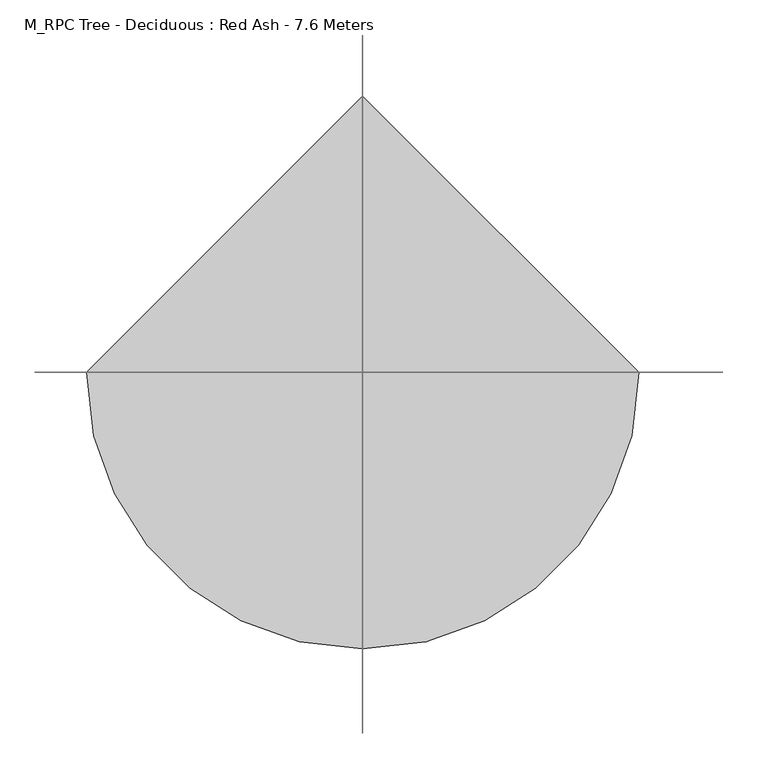
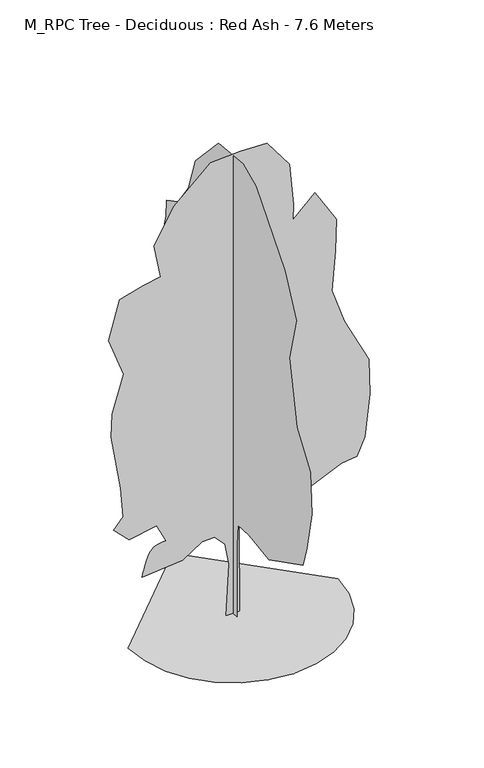
"""IFC4 building model written with IfcOpenShell, lengths in millimetres: geographic element geometry, M_RPC Tree - Deciduous : Red Ash - 7.6 Meters."""

import ifcopenshell
import ifcopenshell.guid

model = None  # the IFC model being written
_history = None  # IfcOwnerHistory: only IFC2X3 demands one
_inside = {}  # id of a spatial element -> (the spatial element, [elements in it])
_under = {}  # id of a project, library or spatial element -> (it, [spatial elements below it])
_declared = {}  # id of a project -> (the project, [libraries it declares])
_typed = {}  # id of a type object -> (the type object, [elements of that type])
_made_of = {}  # id of a material, layer set ... -> (it, [elements and type objects made of it])


def new_model(schema):
    """Start an empty IFC model of exactly this schema.

    Asked for "IFC4X3", IfcOpenShell would pick the latest addendum, in which some entities
    have other attributes; the version numbers below select the first issue.
    IFC2X3 requires an IfcOwnerHistory on every rooted entity: one is made here for all.
    """
    global model, _history
    if schema == "IFC4X3":
        model = ifcopenshell.file(schema_version=(4, 3, 0, 0))
    else:
        model = ifcopenshell.file(schema=schema)
    _inside.clear()
    _under.clear()
    _declared.clear()
    _typed.clear()
    _made_of.clear()
    _history = None
    if model.schema == "IFC2X3":
        org = make("IfcOrganization", Name="unknown")
        user = make(
            "IfcPersonAndOrganization",
            ThePerson=make("IfcPerson", FamilyName="unknown"),
            TheOrganization=org,
        )
        app = make(
            "IfcApplication",
            ApplicationDeveloper=org,
            Version="unknown",
            ApplicationFullName="unknown",
            ApplicationIdentifier="unknown",
        )
        _history = make(
            "IfcOwnerHistory",
            OwningUser=user,
            OwningApplication=app,
            ChangeAction="ADDED",
            CreationDate=0,
        )
    return model


def make(cls, **values):
    """One entity of the class cls with the attributes given. An attribute that is None is left unset."""
    return model.create_entity(
        cls, **{name: value for name, value in values.items() if value is not None}
    )


def rooted(cls, **values):
    """An entity with a GlobalId (a new one), such as an element, a storey or a relation."""
    return make(cls, GlobalId=ifcopenshell.guid.new(), OwnerHistory=_history, **values)


def si_unit(unit_type, name, prefix=None):
    """IfcSIUnit, for example si_unit("LENGTHUNIT", "METRE", prefix="MILLI")."""
    return make("IfcSIUnit", UnitType=unit_type, Prefix=prefix, Name=name)


def assignment(units):
    """IfcUnitAssignment: the units of a project."""
    return None if units is None else make("IfcUnitAssignment", Units=units)


def point(xyz):
    """IfcCartesianPoint."""
    return None if xyz is None else make("IfcCartesianPoint", Coordinates=xyz)


def direction(xyz):
    """IfcDirection."""
    return None if xyz is None else make("IfcDirection", DirectionRatios=xyz)


def frame(location, z_axis=None, x_axis=None):
    """IfcAxis2Placement3D, a coordinate frame: its origin and axes. An axis left out is left unset."""
    return make(
        "IfcAxis2Placement3D",
        Location=point(location),
        Axis=direction(z_axis),
        RefDirection=direction(x_axis),
    )


def origin():
    """The frame at (0, 0, 0) with its axes left unset."""
    return frame((0.0, 0.0, 0.0))


def place(relative_to, where):
    """IfcLocalPlacement: puts the frame where relative to a parent placement (None: the world)."""
    return make(
        "IfcLocalPlacement", PlacementRelTo=relative_to, RelativePlacement=where
    )


def context(
    kind, dimensions, precision=None, world=None, true_north=None, identifier=None
):
    """IfcGeometricRepresentationContext, for example the 3D "Model" context."""
    return make(
        "IfcGeometricRepresentationContext",
        ContextIdentifier=identifier,
        ContextType=kind,
        CoordinateSpaceDimension=dimensions,
        Precision=precision,
        WorldCoordinateSystem=world,
        TrueNorth=true_north,
    )


def project(units=None, contexts=None):
    """IfcProject with its units and contexts."""
    return rooted(
        "IfcProject",
        Name="project",
        RepresentationContexts=contexts,
        UnitsInContext=assignment(units),
    )


def spatial(cls, under=None, at=None, **own):
    """A site, building, storey or space (cls), placed at a placement, below another one or the project."""
    s = rooted(cls, ObjectPlacement=at, **own)
    if under is not None:
        _under.setdefault(under.id(), (under, []))[1].append(s)
    return s


def point_list(points):
    """IfcCartesianPointList2D or 3D."""
    cls = (
        "IfcCartesianPointList2D" if len(points[0]) == 2 else "IfcCartesianPointList3D"
    )
    return make(cls, CoordList=points)


def triangles(points, corners, closed=None, point_numbers=None):
    """IfcTriangulatedFaceSet: each triangle names its three corners, points numbered from 1."""
    return make(
        "IfcTriangulatedFaceSet",
        Coordinates=point_list(points),
        Closed=closed,
        CoordIndex=corners,
        PnIndex=point_numbers,
    )


def shape(context_of_items, identifier, shape_type, items):
    """IfcShapeRepresentation: the items that make up one representation, for example the "Body"."""
    return make(
        "IfcShapeRepresentation",
        ContextOfItems=context_of_items,
        RepresentationIdentifier=identifier,
        RepresentationType=shape_type,
        Items=items,
    )


def source(mapping_origin, context_of_items, identifier, shape_type, items):
    """IfcRepresentationMap: a shape defined once, which mapped items show again and again."""
    return make(
        "IfcRepresentationMap",
        MappingOrigin=mapping_origin,
        MappedRepresentation=shape(context_of_items, identifier, shape_type, items),
    )


def transform(
    local_origin,
    x_axis=None,
    y_axis=None,
    z_axis=None,
    scale=None,
    scale2=None,
    scale3=None,
    uniform=True,
):
    """IfcCartesianTransformationOperator3D, or its non-uniform kind. x_axis, y_axis, z_axis: its Axis1, 2, 3."""
    if uniform:
        return make(
            "IfcCartesianTransformationOperator3D",
            Axis1=direction(x_axis),
            Axis2=direction(y_axis),
            LocalOrigin=point(local_origin),
            Scale=scale,
            Axis3=direction(z_axis),
        )
    return make(
        "IfcCartesianTransformationOperator3DnonUniform",
        Axis1=direction(x_axis),
        Axis2=direction(y_axis),
        LocalOrigin=point(local_origin),
        Scale=scale,
        Axis3=direction(z_axis),
        Scale2=scale2,
        Scale3=scale3,
    )


def mapped(mapping_source, mapping_target):
    """IfcMappedItem: shows the shape of a source again, moved by a transform."""
    return make(
        "IfcMappedItem", MappingSource=mapping_source, MappingTarget=mapping_target
    )


def made_of(thing, what):
    """Note that an element or type object is made of a material, layer set ...; save() writes the relation."""
    if what is not None:
        _made_of.setdefault(what.id(), (what, []))[1].append(thing)
    return thing


def element(
    cls,
    number,
    at=None,
    inside=None,
    cuts=None,
    type_object=None,
    material=None,
    context=None,
    identifier="Body",
    shape_type=None,
    held_by="IfcProductDefinitionShape",
    body=None,
    shapes=None,
    **own,
):
    """One element of the class cls, such as IfcWall. Its Tag is "e" and its number.

    at: its placement. inside: the storey or other place that contains it. cuts: it is an
    opening in that element (IfcRelVoidsElement). A single representation is given by context,
    identifier, shape_type and body (its items); several are given by shapes. held_by: the class
    of the entity that holds the representations. save() writes the other relations.
    """
    e = rooted(cls, Tag="e%d" % number, ObjectPlacement=at, **own)
    if body is not None:
        shapes = [shape(context, identifier, shape_type, body)]
    if shapes is not None:
        e.Representation = make(held_by, Representations=shapes)
    if inside is not None:
        _inside.setdefault(inside.id(), (inside, []))[1].append(e)
    if cuts is not None:
        rooted(
            "IfcRelVoidsElement", RelatingBuildingElement=cuts, RelatedOpeningElement=e
        )
    if type_object is not None:
        _typed.setdefault(type_object.id(), (type_object, []))[1].append(e)
    return made_of(e, material)


def aggregate(whole, parts):
    """IfcRelAggregates: a whole, such as a stair, and the parts it consists of."""
    return rooted("IfcRelAggregates", RelatingObject=whole, RelatedObjects=parts)


def save(model, path):
    """Write the relations noted so far, then the file.

    IfcRelAggregates (storeys below a building ...), IfcRelContainedInSpatialStructure (elements
    in a storey), IfcRelDefinesByType, IfcRelAssociatesMaterial and IfcRelDeclares: one each for
    every whole, place, type object, material and project.
    """
    for whole, parts in _under.values():
        aggregate(whole, parts)
    for where, things in _inside.values():
        rooted(
            "IfcRelContainedInSpatialStructure",
            RelatedElements=things,
            RelatingStructure=where,
        )
    for kind, things in _typed.values():
        rooted("IfcRelDefinesByType", RelatedObjects=things, RelatingType=kind)
    for what, things in _made_of.values():
        rooted("IfcRelAssociatesMaterial", RelatedObjects=things, RelatingMaterial=what)
    for by, libraries in _declared.values():
        rooted("IfcRelDeclares", RelatingContext=by, RelatedDefinitions=libraries)
    model.write(path)


def m_rpc_tree_deciduous_red_ash_7_6_meters_40acba24(model_context):
    return source(origin(), model_context, "Body", "Tessellation", [
        triangles([(-1640.6350319, 0.0, 6.17e-05), (-1597.2618073, -375.9250917, 6.17e-05), (-1473.7362076, -721.1521299, 6.17e-05), (-1279.9481815, -1025.7899305, 6.17e-05), (-1025.7900759, -1279.9483269, 6.17e-05), (-721.1519119, -1473.7357716, 6.17e-05), (-375.9249101, -1597.2618073, 6.17e-05), (7.17e-05, -1640.6350319, 6.17e-05), (375.9250917, -1597.2619526, 6.17e-05), (721.1521299, -1473.7360622, 6.17e-05), (1025.7900759, -1279.9481815, 6.17e-05), (1279.9486176, -1025.7900759, 6.17e-05), (1473.7359169, -721.1519119, 6.17e-05), (1597.2618073, -375.9248374, 6.17e-05), (1640.6350319, 0.0001434, 6.17e-05), (-0.0002151, 1640.6350319, 6.17e-05), (-1.07e-05, -102.5763152, 0.0), (2.5e-05, -100.9809819, 1191.4187742), (3.22e-05, -129.5410573, 1533.7667004), (7e-07, -437.6736119, 1554.0757805), (-5.76e-05, -973.8285673, 1474.4268631), (-0.0001401, -1898.6961697, 1943.5624718), (-0.0001409, -2005.9272697, 2292.063438), (-0.0001357, -2139.9660358, 2935.4496025), (-0.0001116, -2099.7546822, 3605.6435783), (-5.8e-05, -1735.814106, 4130.1484818), (-5.5e-06, -1523.3897175, 5147.0898972), (-3.5e-06, -1711.0423622, 5870.899205), (4.78e-05, -1402.7536217, 6514.2855148), (0.0001565, -625.3287638, 7439.1534805), (0.000198, -272.4836404, 7598.1990051), (0.0002655, 393.3664327, 7532.9808929), (0.0003113, 1023.3488731, 6862.7869171), (0.0003141, 1211.0034073, 6299.8236053), (0.0003314, 1492.4837551, 5897.7074524), (0.0003588, 1800.7742397, 5736.8608749), (0.0003522, 1814.1780727, 5468.7830521), (0.0003514, 1894.6015068, 5160.4937302), (0.0003267, 1760.5627407, 4798.5893669), (0.0003288, 1881.1976738, 4450.088546), (0.000327, 2001.8324615, 3967.5488136), (0.0003203, 1975.0247955, 3833.5096115), (0.0002869, 1747.159053, 3511.8164566), (0.0002722, 1732.7516476, 3069.4885139), (0.0002625, 1720.3510963, 2788.0068581), (0.0002535, 1733.7549294, 2439.5063278), (0.0002406, 1747.159053, 1956.9668861), (0.0002166, 1559.5046642, 1809.523851), (0.0001802, 1211.0038433, 1809.523851), (0.0001822, 1371.8504208, 1313.580431), (0.0001711, 1344.9556961, 1032.1683203), (0.0001512, 1100.1359739, 1224.6137684), (9.84e-05, 627.810589, 1103.8028286), (9.77e-05, 550.2637599, 1353.49907), (6.27e-05, 215.346067, 1350.4488201), (5.01e-05, 130.4579254, 1225.1105404), (3.26e-05, 79.3405423, 816.1354311), (1.17e-05, 111.8716144, 1.28e-05), (-110.5798692, 4.8e-06, 4.45e-05), (-66.5363775, -9.62e-05, 831.3140104), (-128.9679092, -0.0001356, 1184.825572), (-290.0246482, -0.0001497, 1361.7341778), (-482.3670685, -0.0001405, 1355.1302204), (-794.1779051, -0.0001027, 1152.7338535), (-1424.1603092, -6.88e-05, 1099.1184488), (-1415.4458702, -7.33e-05, 1133.781086), (-1406.1451298, -7.8e-05, 1169.6158899), (-1395.6722225, -8.3e-05, 1207.7952456), (-1383.4407017, -8.85e-05, 1249.4921917), (-1368.8645565, -9.46e-05, 1295.8774418), (-1351.3574856, -0.0001016, 1348.1257061), (-1330.3333328, -0.0001096, 1407.4074074), (-1303.8382931, -0.0001173, 1462.3908245), (-1271.0123898, -0.0001236, 1502.6024689), (-1232.9109364, -0.0001286, 1530.5039635), (-1190.588883, -0.0001326, 1548.5586754), (-1145.1018339, -0.0001358, 1559.2267742), (-1097.5041578, -0.0001386, 1564.971191), (-1048.8515316, -0.0001411, 1568.2539848), (-1196.294058, -0.0001698, 1863.1393284), (-1625.218531, -0.0001415, 1782.7160397), (-1866.4879612, -0.0001597, 2023.9863419), (-1719.0452168, -0.0001869, 2198.236607), (-1759.2568611, -0.0002427, 2680.7764847), (-1906.6994602, -0.0003433, 3578.8359123), (-1893.4979404, -0.0003882, 3950.7687332), (-1715.4032879, -0.0004676, 4551.3483536), (-1946.9112499, -0.0005333, 5187.3013962), (-1772.6605488, -0.0006144, 5803.88004), (-1410.7561855, -0.000643, 5911.1112854), (-1135.4252443, -0.0006608, 5959.6792511), (-1236.5059204, -0.0007209, 6500.8816818), (-928.2163805, -0.0007999, 7050.4411606), (-351.8493811, -0.0008874, 7573.192392), (117.2860368, -0.0009111, 7600.000058), (532.8066133, -0.0009277, 7586.5956436), (881.3074705, -0.000887, 7117.4603256), (945.3842279, -0.0008079, 6430.5952744), (936.1832634, -0.0007775, 6178.7100677), (1283.4236961, -0.0008311, 6500.8816818), (1618.5208294, -0.0007802, 5951.3222031), (1605.1169964, -0.0007177, 5432.2143539), (1545.3907001, -0.0006383, 4788.0519287), (1739.1557625, -0.0005793, 4222.2222221), (2126.1689129, -0.0005054, 3460.0925789), (2138.5076946, -0.0004374, 2885.2169128), (2060.848772, -0.0003521, 2198.2364616), (1940.213839, -0.0003133, 1916.7548058), (1698.9439728, -0.0002996, 1889.9471397), (1229.8082188, -0.0002535, 1675.4849396), (814.2876514, -0.0002002, 1380.5997414), (256.8007496, -0.0002044, 1620.3048775), (92.8066444, -0.0001762, 1443.8352711), (103.8818677, -4.5e-06, 3.51e-05)], [[15, 16, 1], [14, 15, 1], [14, 1, 2], [13, 14, 2], [13, 2, 3], [13, 3, 4], [12, 13, 4], [11, 12, 4], [11, 4, 5], [11, 5, 6], [11, 6, 7], [11, 7, 8], [11, 8, 9], [11, 9, 10], [50, 51, 52], [57, 58, 17], [57, 17, 18], [56, 57, 18], [56, 18, 19], [55, 56, 19], [49, 50, 52], [52, 53, 54], [49, 52, 54], [35, 36, 37], [46, 47, 48], [46, 48, 49], [21, 22, 23], [20, 21, 23], [20, 23, 24], [20, 24, 25], [20, 25, 26], [19, 20, 26], [19, 26, 27], [45, 46, 49], [31, 32, 33], [30, 31, 33], [29, 30, 33], [29, 33, 34], [28, 29, 34], [27, 28, 34], [19, 27, 34], [19, 34, 35], [19, 35, 37], [19, 37, 38], [19, 38, 39], [19, 39, 40], [19, 40, 41], [19, 41, 42], [19, 42, 43], [19, 43, 44], [19, 44, 45], [19, 45, 49], [19, 49, 54], [55, 19, 54], [64, 65, 66], [64, 66, 67], [64, 67, 68], [99, 100, 101], [64, 68, 69], [64, 69, 70], [64, 70, 71], [114, 59, 60], [113, 114, 60], [113, 60, 61], [113, 61, 62], [64, 71, 72], [64, 72, 73], [64, 73, 74], [64, 74, 75], [64, 75, 76], [64, 76, 77], [64, 77, 78], [64, 78, 79], [63, 64, 79], [81, 82, 83], [80, 81, 83], [99, 101, 102], [107, 108, 109], [110, 111, 112], [88, 89, 90], [87, 88, 90], [87, 90, 91], [80, 83, 84], [95, 96, 97], [95, 97, 98], [94, 95, 98], [93, 94, 98], [92, 93, 98], [91, 92, 98], [91, 98, 99], [87, 91, 99], [87, 99, 102], [87, 102, 103], [87, 103, 104], [86, 87, 104], [85, 86, 104], [84, 85, 104], [80, 84, 104], [80, 104, 105], [80, 105, 106], [80, 106, 107], [80, 107, 109], [80, 109, 110], [80, 110, 112], [79, 80, 112], [63, 79, 112], [62, 63, 112], [113, 62, 112]], closed=False),
    ])


if __name__ == "__main__":
    model = new_model("IFC4")
    model_context = context("Model", 3, world=origin())
    ifc_project = project(units=[si_unit("LENGTHUNIT", "METRE", prefix="MILLI")], contexts=[model_context])
    site = spatial("IfcSite", under=ifc_project)
    building = spatial("IfcBuilding", under=site)
    placement = place(None, origin())
    m_rpc_tree_deciduous_red_ash_7_6_meters_shape = m_rpc_tree_deciduous_red_ash_7_6_meters_40acba24(model_context)
    element("IfcGeographicElement", 1, ObjectType="M_RPC Tree - Deciduous : Red Ash - 7.6 Meters", at=placement, inside=building, context=model_context, shape_type="MappedRepresentation", body=[
        mapped(m_rpc_tree_deciduous_red_ash_7_6_meters_shape, transform((0.0, 0.0, 0.0), x_axis=(1.0, 0.0, 0.0), y_axis=(0.0, 1.0, 0.0), z_axis=(0.0, 0.0, 1.0))),
    ])
    save(model, "model.ifc")

# Revit data of these elements
# Type "M_RPC Tree - Deciduous : Red Ash - 7.6 Meters"
#   built-in parameter 1005198 = "{2, 15},{22, RPC-8-G3GR-497X-PHW5-6},{1, 0},{1, 0},{2, 15},{1, 8},{5, Color},{1, 0},{1, 0},{3, 0.8},{3, 0.8},{3, 0.8},{1, 8},{7, BBoxMin},{1, 0},{1, 0},{1, 0},{1, 0},{1, 0},{1, 8},{7, BBoxMax},{1, 0},{1, 0},{1, 0},{1, 0},{1, 0},{2, 11},{9, RPCTypeId},{1, 0},{1, 0},{22, RPC-8-G3GR-497X-PHW5-6},{1, 6},{14, RPCPlantHeight},{1, 0},{1, 0},{7, 24.9344},{2, 11},{7, keyword},{1, 0},{1, 0},{34, :RPCs:Trees [General]:Geometry:RPC},{2, 11},{8, category},{1, 0},{1, 0},{15, Trees [General]},{2, 11},{12, LocalizedUID},{1, 0},{1, 0},{7, Red Ash},{2, 14},{6, Height},{1, 0},{1, 0},{7, 24.9344},{1, 2},{16, Cast Reflections},{1, 0},{1, 0},{1, 0},{1, 2},{6, Jitter},{1, 0},{1, 0},{1, 1},{1, 2},{9, Billboard},{1, 0},{1, 0},{1, 0},{1, 2},{12, Cast Shadows},{1, 0},{1, 0},{1, 1},{1, 2},{20, Apply Filter Effects},{1, 0},{1, 0},{1, 0},{2, 11},{28, Apply Filter Effects-Text-FC},{1, 0},{1, 0},{4, None},{21, assetlibrary_base.fbx},{1, 5},"
#   built-in parameter 1005195 = "RPC-8-G3GR-497X-PHW5-6"
#   Type Comments = "Red Ash"
#   Height = 7.600 m
#   Default Elevation = 0
